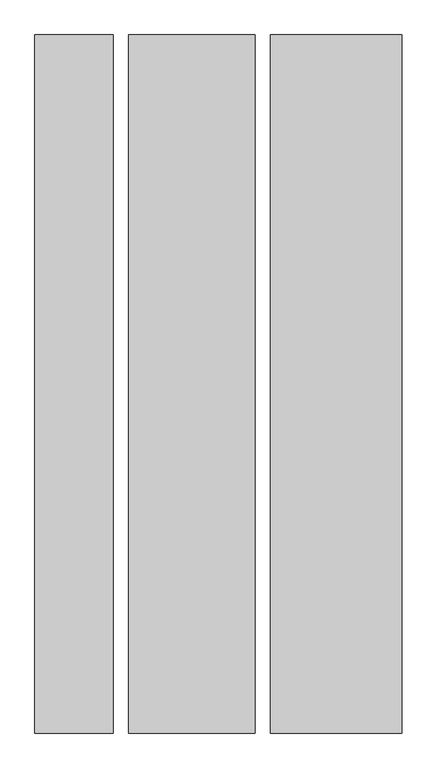
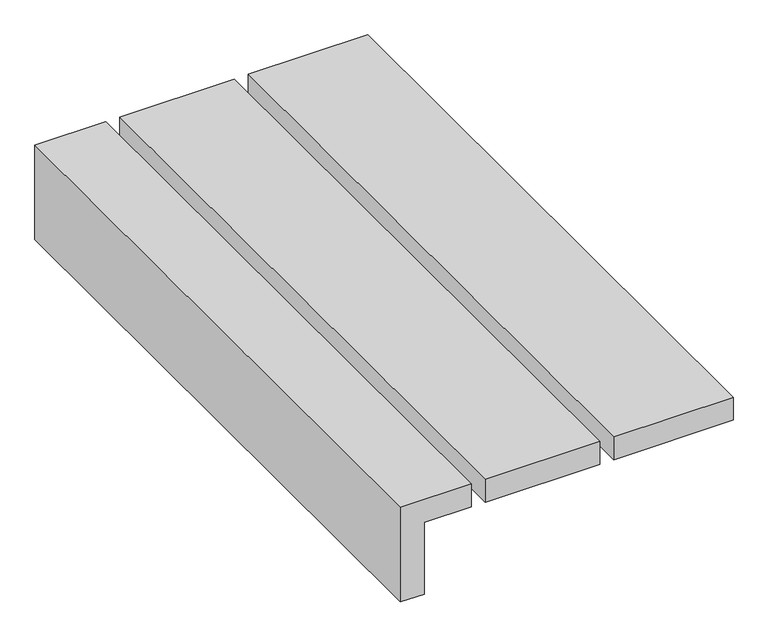
"""IFC4 building model written with IfcOpenShell, lengths in millimetres: proxy geometry, Blocking106 12412 : Blocking106 12412."""

import ifcopenshell
import ifcopenshell.guid

model = None  # the IFC model being written
_history = None  # IfcOwnerHistory: only IFC2X3 demands one
_inside = {}  # id of a spatial element -> (the spatial element, [elements in it])
_under = {}  # id of a project, library or spatial element -> (it, [spatial elements below it])
_declared = {}  # id of a project -> (the project, [libraries it declares])
_typed = {}  # id of a type object -> (the type object, [elements of that type])
_made_of = {}  # id of a material, layer set ... -> (it, [elements and type objects made of it])


def new_model(schema):
    """Start an empty IFC model of exactly this schema.

    Asked for "IFC4X3", IfcOpenShell would pick the latest addendum, in which some entities
    have other attributes; the version numbers below select the first issue.
    IFC2X3 requires an IfcOwnerHistory on every rooted entity: one is made here for all.
    """
    global model, _history
    if schema == "IFC4X3":
        model = ifcopenshell.file(schema_version=(4, 3, 0, 0))
    else:
        model = ifcopenshell.file(schema=schema)
    _inside.clear()
    _under.clear()
    _declared.clear()
    _typed.clear()
    _made_of.clear()
    _history = None
    if model.schema == "IFC2X3":
        org = make("IfcOrganization", Name="unknown")
        user = make(
            "IfcPersonAndOrganization",
            ThePerson=make("IfcPerson", FamilyName="unknown"),
            TheOrganization=org,
        )
        app = make(
            "IfcApplication",
            ApplicationDeveloper=org,
            Version="unknown",
            ApplicationFullName="unknown",
            ApplicationIdentifier="unknown",
        )
        _history = make(
            "IfcOwnerHistory",
            OwningUser=user,
            OwningApplication=app,
            ChangeAction="ADDED",
            CreationDate=0,
        )
    return model


def make(cls, **values):
    """One entity of the class cls with the attributes given. An attribute that is None is left unset."""
    return model.create_entity(
        cls, **{name: value for name, value in values.items() if value is not None}
    )


def rooted(cls, **values):
    """An entity with a GlobalId (a new one), such as an element, a storey or a relation."""
    return make(cls, GlobalId=ifcopenshell.guid.new(), OwnerHistory=_history, **values)


def si_unit(unit_type, name, prefix=None):
    """IfcSIUnit, for example si_unit("LENGTHUNIT", "METRE", prefix="MILLI")."""
    return make("IfcSIUnit", UnitType=unit_type, Prefix=prefix, Name=name)


def assignment(units):
    """IfcUnitAssignment: the units of a project."""
    return None if units is None else make("IfcUnitAssignment", Units=units)


def point(xyz):
    """IfcCartesianPoint."""
    return None if xyz is None else make("IfcCartesianPoint", Coordinates=xyz)


def direction(xyz):
    """IfcDirection."""
    return None if xyz is None else make("IfcDirection", DirectionRatios=xyz)


def frame(location, z_axis=None, x_axis=None):
    """IfcAxis2Placement3D, a coordinate frame: its origin and axes. An axis left out is left unset."""
    return make(
        "IfcAxis2Placement3D",
        Location=point(location),
        Axis=direction(z_axis),
        RefDirection=direction(x_axis),
    )


def origin():
    """The frame at (0, 0, 0) with its axes left unset."""
    return frame((0.0, 0.0, 0.0))


def place(relative_to, where):
    """IfcLocalPlacement: puts the frame where relative to a parent placement (None: the world)."""
    return make(
        "IfcLocalPlacement", PlacementRelTo=relative_to, RelativePlacement=where
    )


def context(
    kind, dimensions, precision=None, world=None, true_north=None, identifier=None
):
    """IfcGeometricRepresentationContext, for example the 3D "Model" context."""
    return make(
        "IfcGeometricRepresentationContext",
        ContextIdentifier=identifier,
        ContextType=kind,
        CoordinateSpaceDimension=dimensions,
        Precision=precision,
        WorldCoordinateSystem=world,
        TrueNorth=true_north,
    )


def project(units=None, contexts=None):
    """IfcProject with its units and contexts."""
    return rooted(
        "IfcProject",
        Name="project",
        RepresentationContexts=contexts,
        UnitsInContext=assignment(units),
    )


def spatial(cls, under=None, at=None, **own):
    """A site, building, storey or space (cls), placed at a placement, below another one or the project."""
    s = rooted(cls, ObjectPlacement=at, **own)
    if under is not None:
        _under.setdefault(under.id(), (under, []))[1].append(s)
    return s


def polyline(points):
    """IfcPolyline through the points."""
    return make("IfcPolyline", Points=[point(p) for p in points])


def outline(outer, holes=None, kind="AREA"):
    """IfcArbitraryClosedProfileDef: a profile drawn as a closed curve; with holes, ...WithVoids."""
    if holes is None:
        return make("IfcArbitraryClosedProfileDef", ProfileType=kind, OuterCurve=outer)
    return make(
        "IfcArbitraryProfileDefWithVoids",
        ProfileType=kind,
        OuterCurve=outer,
        InnerCurves=holes,
    )


def extrude(swept, where, along, depth):
    """IfcExtrudedAreaSolid: the profile swept, set in the frame where, extruded along a direction by depth."""
    return make(
        "IfcExtrudedAreaSolid",
        SweptArea=swept,
        Position=where,
        ExtrudedDirection=direction(along),
        Depth=depth,
    )


def shape(context_of_items, identifier, shape_type, items):
    """IfcShapeRepresentation: the items that make up one representation, for example the "Body"."""
    return make(
        "IfcShapeRepresentation",
        ContextOfItems=context_of_items,
        RepresentationIdentifier=identifier,
        RepresentationType=shape_type,
        Items=items,
    )


def source(mapping_origin, context_of_items, identifier, shape_type, items):
    """IfcRepresentationMap: a shape defined once, which mapped items show again and again."""
    return make(
        "IfcRepresentationMap",
        MappingOrigin=mapping_origin,
        MappedRepresentation=shape(context_of_items, identifier, shape_type, items),
    )


def transform(
    local_origin,
    x_axis=None,
    y_axis=None,
    z_axis=None,
    scale=None,
    scale2=None,
    scale3=None,
    uniform=True,
):
    """IfcCartesianTransformationOperator3D, or its non-uniform kind. x_axis, y_axis, z_axis: its Axis1, 2, 3."""
    if uniform:
        return make(
            "IfcCartesianTransformationOperator3D",
            Axis1=direction(x_axis),
            Axis2=direction(y_axis),
            LocalOrigin=point(local_origin),
            Scale=scale,
            Axis3=direction(z_axis),
        )
    return make(
        "IfcCartesianTransformationOperator3DnonUniform",
        Axis1=direction(x_axis),
        Axis2=direction(y_axis),
        LocalOrigin=point(local_origin),
        Scale=scale,
        Axis3=direction(z_axis),
        Scale2=scale2,
        Scale3=scale3,
    )


def mapped(mapping_source, mapping_target):
    """IfcMappedItem: shows the shape of a source again, moved by a transform."""
    return make(
        "IfcMappedItem", MappingSource=mapping_source, MappingTarget=mapping_target
    )


def made_of(thing, what):
    """Note that an element or type object is made of a material, layer set ...; save() writes the relation."""
    if what is not None:
        _made_of.setdefault(what.id(), (what, []))[1].append(thing)
    return thing


def element(
    cls,
    number,
    at=None,
    inside=None,
    cuts=None,
    type_object=None,
    material=None,
    context=None,
    identifier="Body",
    shape_type=None,
    held_by="IfcProductDefinitionShape",
    body=None,
    shapes=None,
    **own,
):
    """One element of the class cls, such as IfcWall. Its Tag is "e" and its number.

    at: its placement. inside: the storey or other place that contains it. cuts: it is an
    opening in that element (IfcRelVoidsElement). A single representation is given by context,
    identifier, shape_type and body (its items); several are given by shapes. held_by: the class
    of the entity that holds the representations. save() writes the other relations.
    """
    e = rooted(cls, Tag="e%d" % number, ObjectPlacement=at, **own)
    if body is not None:
        shapes = [shape(context, identifier, shape_type, body)]
    if shapes is not None:
        e.Representation = make(held_by, Representations=shapes)
    if inside is not None:
        _inside.setdefault(inside.id(), (inside, []))[1].append(e)
    if cuts is not None:
        rooted(
            "IfcRelVoidsElement", RelatingBuildingElement=cuts, RelatedOpeningElement=e
        )
    if type_object is not None:
        _typed.setdefault(type_object.id(), (type_object, []))[1].append(e)
    return made_of(e, material)


def aggregate(whole, parts):
    """IfcRelAggregates: a whole, such as a stair, and the parts it consists of."""
    return rooted("IfcRelAggregates", RelatingObject=whole, RelatedObjects=parts)


def save(model, path):
    """Write the relations noted so far, then the file.

    IfcRelAggregates (storeys below a building ...), IfcRelContainedInSpatialStructure (elements
    in a storey), IfcRelDefinesByType, IfcRelAssociatesMaterial and IfcRelDeclares: one each for
    every whole, place, type object, material and project.
    """
    for whole, parts in _under.values():
        aggregate(whole, parts)
    for where, things in _inside.values():
        rooted(
            "IfcRelContainedInSpatialStructure",
            RelatedElements=things,
            RelatingStructure=where,
        )
    for kind, things in _typed.values():
        rooted("IfcRelDefinesByType", RelatedObjects=things, RelatingType=kind)
    for what, things in _made_of.values():
        rooted("IfcRelAssociatesMaterial", RelatedObjects=things, RelatingMaterial=what)
    for by, libraries in _declared.values():
        rooted("IfcRelDeclares", RelatingContext=by, RelatedDefinitions=libraries)
    model.write(path)


def generic_models_2ceb33a1(model_context):
    return source(origin(), model_context, "Body", "SweptSolid", [
        extrude(outline(polyline([(44042.7623529, 6172.6163563), (44042.7623529, 6320.6984495), (44118.9623529, 6320.6984495), (44118.9623529, 6096.4163563), (43803.0227817, 6096.4163563), (43803.0227817, 6172.6163563), (44042.7623529, 6172.6163563)])), frame((0.0, -1052.8908936, 0.0), z_axis=(0.0, 1.0, 0.0), x_axis=(0.0, 0.0, 1.0)), (0.0, 0.0, 1.0), 2000.0),
        extrude(outline(polyline([(7149.3612048, -1052.8908936), (6771.5484495, -1052.8908936), (6771.5484495, 947.1091064), (7149.3612048, 947.1091064), (7149.3612048, -1052.8908936)])), frame((0.0, 0.0, 44042.7623529), z_axis=(0.0, 0.0, 1.0), x_axis=(1.0, 0.0, 0.0)), (0.0, 0.0, 1.0), 76.2),
        extrude(outline(polyline([(6727.0984495, -1052.8908936), (6365.1484495, -1052.8908936), (6365.1484495, 947.1091064), (6727.0984495, 947.1091064), (6727.0984495, -1052.8908936)])), frame((0.0, 0.0, 44042.7623529), z_axis=(0.0, 0.0, 1.0), x_axis=(1.0, 0.0, 0.0)), (0.0, 0.0, 1.0), 76.2),
    ])


if __name__ == "__main__":
    model = new_model("IFC4")
    model_context = context("Model", 3, world=origin())
    ifc_project = project(units=[si_unit("LENGTHUNIT", "METRE", prefix="MILLI")], contexts=[model_context])
    site = spatial("IfcSite", under=ifc_project)
    building = spatial("IfcBuilding", under=site)
    placement = place(None, origin())
    generic_models_shape = generic_models_2ceb33a1(model_context)
    element("IfcBuildingElementProxy", 1, Name="Blocking106 12412 : Blocking106 12412", ObjectType="Blocking106 12412 : Blocking106 12412", at=placement, inside=building, context=model_context, shape_type="MappedRepresentation", body=[
        mapped(generic_models_shape, transform((0.0, 0.0, 0.0), x_axis=(1.0, 0.0, 0.0), y_axis=(0.0, 1.0, 0.0), z_axis=(0.0, 0.0, 1.0))),
    ])
    save(model, "model.ifc")

# Revit data of these elements
# Type "Blocking106 12412 : Blocking106 12412"
#   NameOverride = "Blocking106"
# Element 1 (IfcBuildingElementProxy, "Blocking106 12412 : Blocking106 12412")
#   Materials on its faces: "POLYURETHANE SPRAY FOAM UNDER ROOF SUBSTRATE (SEE T-24 ENERGY REPORT FOR R-VALUE)"
# Materials
#   "POLYURETHANE SPRAY FOAM UNDER ROOF SUBSTRATE (SEE T-24 ENERGY REPORT FOR R-VALUE)": class "Unassigned", colour RGB 210 164 194, transparency 0, Cost = 0
